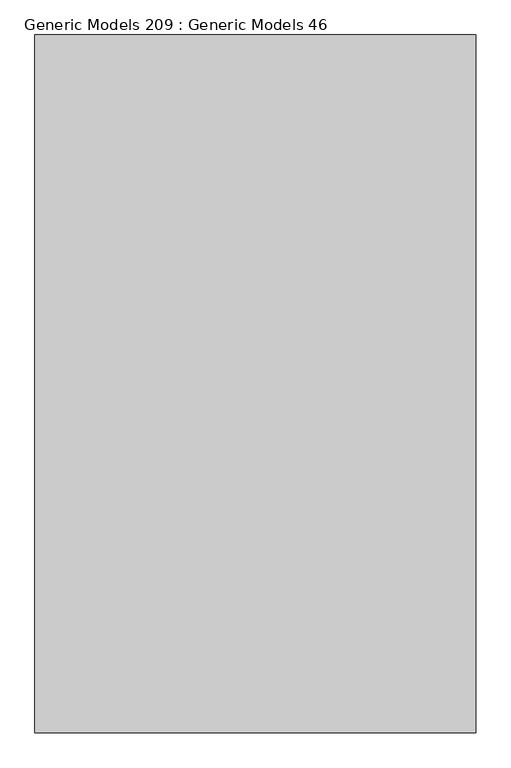
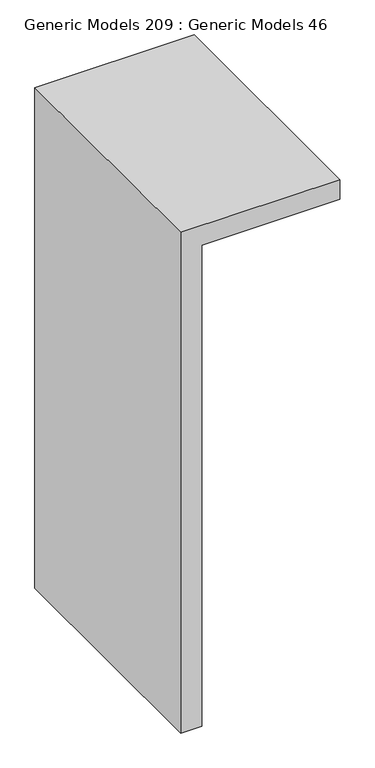
"""IFC4 building model written with IfcOpenShell, lengths in millimetres: proxy geometry, Generic Models 209 : Generic Models 46."""

from ifc_helpers import new_model, si_unit, frame, origin, place, context, project, spatial, polyline, outline, extrude, source, transform, mapped, element, save


def generic_models_209_generic_models_46_b9e04646(model_context):
    return source(origin(), model_context, "Body", "SweptSolid", [
        extrude(outline(polyline([(2559.05, 46689.9625), (2559.05, 45920.025), (0.0, 45920.025), (0.0, 46021.625), (2457.45, 46021.625), (2457.45, 46689.9625), (2559.05, 46689.9625)])), frame((0.0, 0.0, 0.0), z_axis=(0.0, 1.0, 0.0), x_axis=(0.0, 0.0, 1.0)), (0.0, 0.0, 1.0), 1219.2),
    ])


if __name__ == "__main__":
    model = new_model("IFC4")
    model_context = context("Model", 3, world=origin())
    ifc_project = project(units=[si_unit("LENGTHUNIT", "METRE", prefix="MILLI")], contexts=[model_context])
    site = spatial("IfcSite", under=ifc_project)
    building = spatial("IfcBuilding", under=site)
    placement = place(None, origin())
    generic_models_209_generic_models_46_shape = generic_models_209_generic_models_46_b9e04646(model_context)
    element("IfcBuildingElementProxy", 1, Name="Generic Models 209 : Generic Models 46", ObjectType="Generic Models 209 : Generic Models 46", at=placement, inside=building, context=model_context, shape_type="MappedRepresentation", body=[
        mapped(generic_models_209_generic_models_46_shape, transform((0.0, 0.0, 0.0), x_axis=(1.0, 0.0, 0.0), y_axis=(0.0, 1.0, 0.0), z_axis=(0.0, 0.0, 1.0))),
    ])
    save(model, "model.ifc")

# Revit data of these elements
# Element 1 (IfcBuildingElementProxy, "Generic Models 209 : Generic Models 46")
#   Materials on its faces: "EXISTING STRUCTURE"
# Materials
#   "EXISTING STRUCTURE": class "Concrete", colour RGB 36 37 33, transparency 0, Description = "Lightweight concrete", Cost = 0
